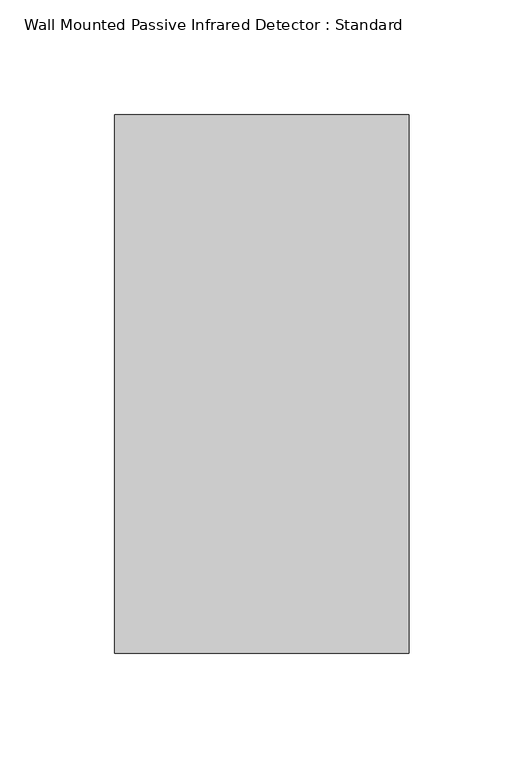
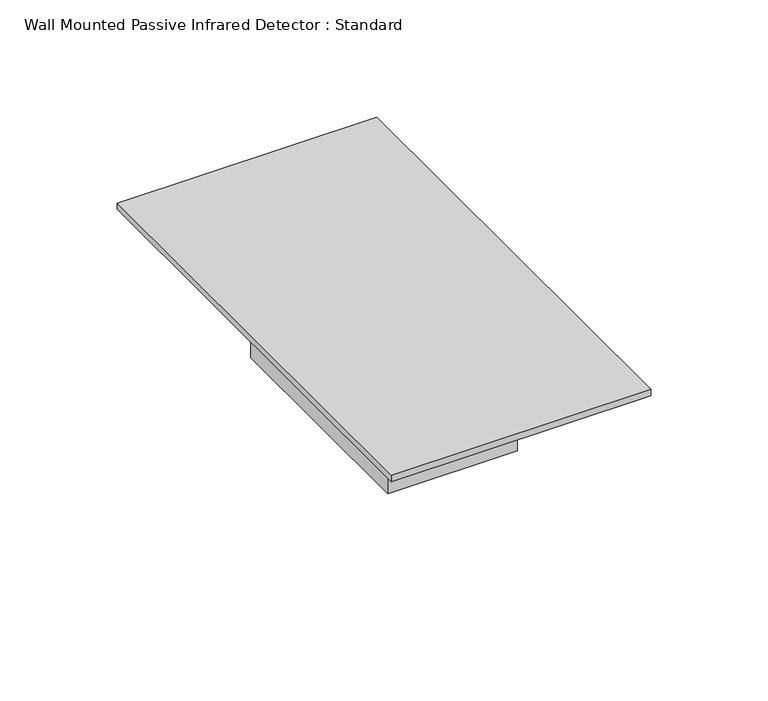
"""IFC4 building model written with IfcOpenShell, lengths in millimetres: proxy geometry, Wall Mounted Passive Infrared Detector : Standard."""

from ifc_helpers import new_model, si_unit, frame, origin, origin_with_axes, place, context, project, spatial, polyline, outline, extrude, source, transform, mapped, element, save


def wall_mounted_passive_infrared_detector_standard_722f1ccb(model_context):
    return source(origin(), model_context, "Body", "SweptSolid", [
        extrude(outline(polyline([(64.0, 0.0), (64.0, -234.0), (-64.0, -234.0), (-64.0, 0.0), (64.0, 0.0)])), origin_with_axes(), (0.0, 0.0, 1.0), 3.3125),
        extrude(outline(polyline([(32.0, -58.5), (32.0, -175.5), (-32.0, -175.5), (-32.0, -58.5), (32.0, -58.5)])), frame((0.0, 0.0, -53.0), z_axis=(0.0, 0.0, 1.0), x_axis=(1.0, 0.0, 0.0)), (0.0, 0.0, 1.0), 53.0),
    ])


if __name__ == "__main__":
    model = new_model("IFC4")
    model_context = context("Model", 3, world=origin())
    ifc_project = project(units=[si_unit("LENGTHUNIT", "METRE", prefix="MILLI")], contexts=[model_context])
    site = spatial("IfcSite", under=ifc_project)
    building = spatial("IfcBuilding", under=site)
    placement = place(None, origin())
    wall_mounted_passive_infrared_detector_standard_shape = wall_mounted_passive_infrared_detector_standard_722f1ccb(model_context)
    element("IfcBuildingElementProxy", 1, Name="Wall Mounted Passive Infrared Detector : Standard", ObjectType="Wall Mounted Passive Infrared Detector : Standard", at=placement, inside=building, context=model_context, shape_type="MappedRepresentation", body=[
        mapped(wall_mounted_passive_infrared_detector_standard_shape, transform((0.0, 0.0, 0.0), x_axis=(1.0, 0.0, 0.0), y_axis=(0.0, 1.0, 0.0), z_axis=(0.0, 0.0, 1.0))),
    ])
    save(model, "model.ifc")

# Revit data of these elements
# Type "Wall Mounted Passive Infrared Detector : Standard"
#   Type Mark = "Wall Mounted Passive Infrared Detector"
#   Classification.OmniClass.21.Number = "21-04 70 70 10"
#   Classification.OmniClass.21.Description = "Electronic Detention Monitoring and Control"
#   Classification.UniFormat.II.Description = "Intruction Detection"
#   Classification.OmniClass.23.Number = "23-29 11 21"
#   Classification.OmniClass.23.Description = "Security Sensors"
#   Classification.UniFormat.II.Number = "D7010.50"
#   COBie.Type.CreatedBy = "info@mma.ie"
#   COBie.Type.CreatedOn = "2017-07-26T09:12:44"
#   COBie.Type.Name = "Wall Mounted Passive Infrared Detector"
#   COBie.Type.Category = "23-29 11 21 : Security Sensors"
#   COBie.Type.Description = "Wall Mounted Passive Infrared Detector_Standard"
#   COBie.Type.AssetType = "Movable"
#   COBie.Type.Manufacturer = ""
#   COBie.Type.ModelNumber = ""
#   COBie.Type.ModelReference = ""
#   COBie.Type.Color = "White"
#   Units = "Volts"
#   Label = "PIR"
#   Keynote = "28 16 19.A"
#   COBie.Type.ReplacementCost = 0
#   Width 1 = 128 mm
#   Sensor Voltage = 230 V
#   PIR_Width = 64 mm
#   PIR_Depth = 53 mm
#   PIR Height = 117 mm
#   Length 1 = 234 mm
#   Height 1 = 3.312 mm
#   Default Elevation = 1200 mm
#   Sensor Width = 64 mm
#   Sensor Length = 117 mm
#   Sensor Height = 53 mm
#   Apparent Load = 0 VA
#   COBie.Type = yes
#   Sensor Number of Poles = 1
#   Sensor Material = none
#   Load Classification = Other
#   Cover Material = none
#   URL = ""
#   Model = ""
#   Manufacturer = ""
